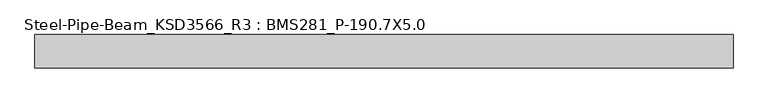
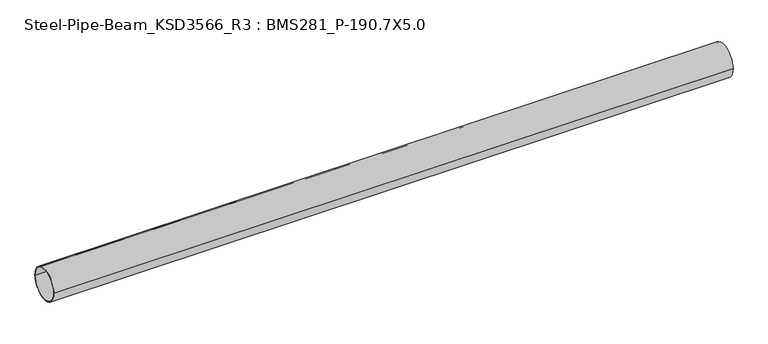
"""IFC4 building model written with IfcOpenShell, lengths in millimetres: member geometry, Steel-Pipe-Beam_KSD3566_R3 : BMS281_P-190.7X5.0."""

from ifc_helpers import new_model, si_unit, point, frame, origin, origin_2d, place, context, project, spatial, circle_curve, trimmed, segment, composite_curve, outline, extrude, source, transform, mapped, element, save


def steel_pipe_beam_ksd3566_r3_bms281_p_190_7x5_0_d9e19f43(model_context):
    return source(origin(), model_context, "Body", "SweptSolid", [
        extrude(outline(composite_curve([segment(trimmed(circle_curve(origin_2d(), 95.35), [point((-95.35, 0.0))], [point((95.35, 0.0))], False, "CARTESIAN"), True, "CONTINUOUS"), segment(trimmed(circle_curve(origin_2d(), 95.35), [point((95.35, 0.0))], [point((-95.35, 0.0))], False, "CARTESIAN"), True, "CONTINUOUS")], self_intersect=False), holes=[composite_curve([segment(trimmed(circle_curve(origin_2d(), 90.35), [point((90.35, 0.0))], [point((-90.35, 0.0))], True, "CARTESIAN"), True, "CONTINUOUS"), segment(trimmed(circle_curve(origin_2d(), 90.35), [point((-90.35, 0.0))], [point((90.35, 0.0))], True, "CARTESIAN"), True, "CONTINUOUS")], self_intersect=False)]), frame((-1979.4197206, 0.0, 0.0), z_axis=(1.0, 0.0, 0.0), x_axis=(0.0, 1.0, 0.0)), (0.0, 0.0, 1.0), 3969.6013202),
    ])


if __name__ == "__main__":
    model = new_model("IFC4")
    model_context = context("Model", 3, world=origin())
    ifc_project = project(units=[si_unit("LENGTHUNIT", "METRE", prefix="MILLI")], contexts=[model_context])
    site = spatial("IfcSite", under=ifc_project)
    building = spatial("IfcBuilding", under=site)
    placement = place(None, origin())
    steel_pipe_beam_ksd3566_r3_bms281_p_190_7x5_0_shape = steel_pipe_beam_ksd3566_r3_bms281_p_190_7x5_0_d9e19f43(model_context)
    element("IfcMember", 1, ObjectType="Steel-Pipe-Beam_KSD3566_R3 : BMS281_P-190.7X5.0", at=placement, inside=building, context=model_context, shape_type="MappedRepresentation", body=[
        mapped(steel_pipe_beam_ksd3566_r3_bms281_p_190_7x5_0_shape, transform((0.0, 0.0, 0.0), x_axis=(1.0, 0.0, 0.0), y_axis=(0.0, 1.0, 0.0), z_axis=(0.0, 0.0, 1.0))),
    ])
    save(model, "model.ifc")

# Revit data of these elements
# Type "Steel-Pipe-Beam_KSD3566_R3 : BMS281_P-190.7X5.0"
#   Keynote = "P-190.7X5.0"
#   SteelWeight = "Light"
#   t = 0.0050 m
#   Surface Area = 0.599102 m²/m
#   Section Area = 29.1697 cm²
#   Mass per Unit Length = 22.8982 kg/m
#   Length [instance default] = 1.5000 m
#   D = 0.1907 m
#   hec_material4 [instance default] = none
#   hec_material3 [instance default] = none
#   hec_material2 [instance default] = none
#   hec_material1 [instance default] = none
#   Structural Material [instance default] = Steel, 45-345
#   Assembly Code = ""
# Element 1 (IfcMember, "Steel-Pipe-Beam_KSD3566_R3 : BMS281_P-190.7X5.0")
#   Structural Material = none
# Materials
#   "Steel, 45-345": class "Metal", colour RGB 189 187 185, transparency 0, Description = "Steel 345 MPa", Cost = 0
